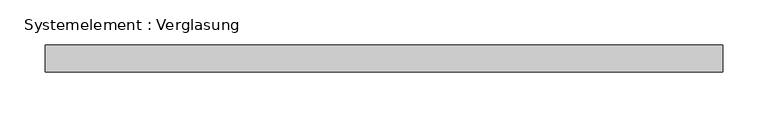
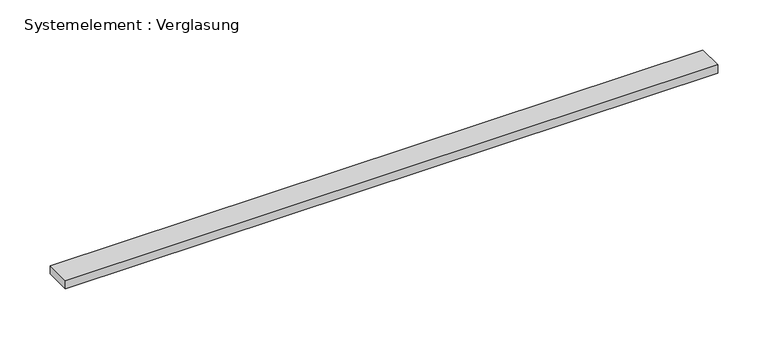
"""IFC4 building model written with IfcOpenShell, lengths in millimetres: plate geometry, Systemelement : Verglasung."""

from ifc_helpers import new_model, si_unit, origin, origin_with_axes, place, context, project, spatial, polyline, outline, extrude, source, transform, mapped, element, save


def systemelement_verglasung_e037e7bf(model_context):
    return source(origin(), model_context, "Body", "SweptSolid", [
        extrude(outline(polyline([(376.4731315, -15.0), (-376.4731315, -15.0), (-376.4731315, 15.0), (376.4731315, 15.0), (376.4731315, -15.0)])), origin_with_axes(), (0.0, 0.0, 1.0), 10.0),
    ])


if __name__ == "__main__":
    model = new_model("IFC4")
    model_context = context("Model", 3, world=origin())
    ifc_project = project(units=[si_unit("LENGTHUNIT", "METRE", prefix="MILLI")], contexts=[model_context])
    site = spatial("IfcSite", under=ifc_project)
    building = spatial("IfcBuilding", under=site)
    placement = place(None, origin())
    systemelement_verglasung_shape = systemelement_verglasung_e037e7bf(model_context)
    element("IfcPlate", 1, ObjectType="Systemelement : Verglasung", at=placement, inside=building, context=model_context, shape_type="MappedRepresentation", body=[
        mapped(systemelement_verglasung_shape, transform((0.0, 0.0, 0.0), x_axis=(1.0, 0.0, 0.0), y_axis=(0.0, 1.0, 0.0), z_axis=(0.0, 0.0, 1.0))),
    ])
    save(model, "model.ifc")

# Revit data of these elements
# Type "Systemelement : Verglasung"
#   Construction Type Id = "GSP4R"
#   Analytic Construction = "1/8 Zoll Pilkington-Verglasung einfach"
#   Visual Light Transmittance = 0.9
#   Solar Heat Gain Coefficient = 0.86
#   Heat Transfer Coefficient (U) = 6.7069 W/(m²·K)
# Element 1 (IfcPlate, "Systemelement : Verglasung")
#   Materials on its faces: "Glas"
# Materials
#   "Glas": class "Glas", colour RGB 0 0 255, transparency 0.75, Comments = "Render-Darstellung nicht aktualisiert ", Cost = 0
